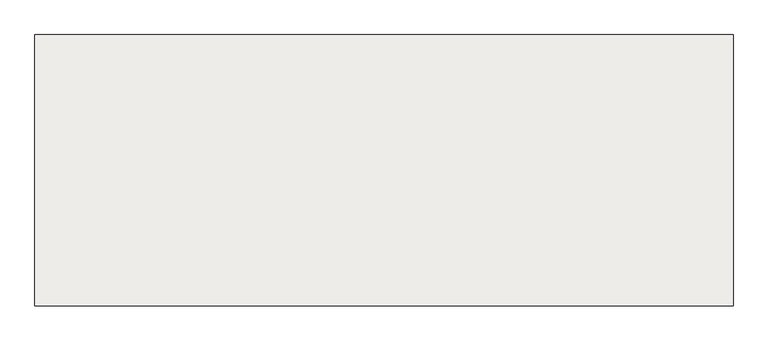
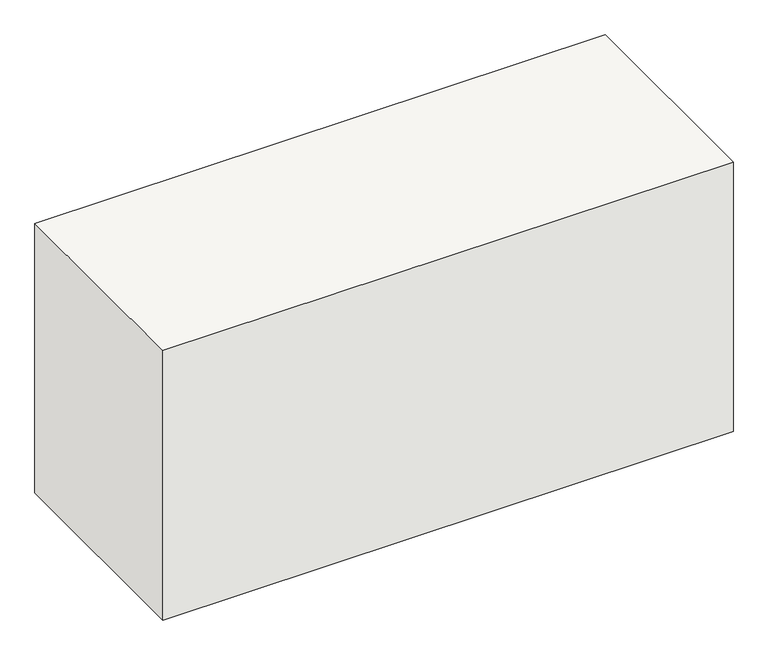
"""IFC4 building model written with IfcOpenShell, lengths in millimetres: footing geometry, NLRS_16_SFO_LB_funderingspoer meerpaals beton ihwg-MMBC-SH_gen_rsf : funderingspoer beton ihwg_gen__2-paals bxlxh 700x1800x1200."""

from ifc_helpers import new_model, si_unit, frame, origin, place, context, project, spatial, polyline, outline, extrude, source, transform, mapped, element, save


def footing_ec8fc613(model_context):
    return source(origin(), model_context, "Body", "SweptSolid", [
        extrude(outline(polyline([(900.0, 350.0), (900.0, -350.0), (-900.0, -350.0), (-900.0, 350.0), (900.0, 350.0)])), frame((0.0, 0.0, -1200.0), z_axis=(0.0, 0.0, 1.0), x_axis=(1.0, 0.0, 0.0)), (0.0, 0.0, 1.0), 900.0),
    ])


if __name__ == "__main__":
    model = new_model("IFC4")
    model_context = context("Model", 3, world=origin())
    ifc_project = project(units=[si_unit("LENGTHUNIT", "METRE", prefix="MILLI")], contexts=[model_context])
    site = spatial("IfcSite", under=ifc_project)
    building = spatial("IfcBuilding", under=site)
    placement = place(None, origin())
    footing_shape = footing_ec8fc613(model_context)
    element("IfcFooting", 1, ObjectType="NLRS_16_SFO_LB_funderingspoer meerpaals beton ihwg-MMBC-SH_gen_rsf : funderingspoer beton ihwg_gen__2-paals bxlxh 700x1800x1200", at=placement, inside=building, context=model_context, shape_type="MappedRepresentation", body=[
        mapped(footing_shape, transform((0.0, 0.0, 0.0), x_axis=(1.0, 0.0, 0.0), y_axis=(0.0, 1.0, 0.0), z_axis=(0.0, 0.0, 1.0))),
    ])
    save(model, "model.ifc")

# Revit data of these elements
# Type "NLRS_16_SFO_LB_funderingspoer meerpaals beton ihwg-MMBC-SH_gen_rsf : funderingspoer beton ihwg_gen__2-paals bxlxh 700x1800x1200"
#   IfcExportAs = "IfcFootingType"
#   Type Comments = "2-paals poer 700x1800x1200"
#   Model = " "
#   Manufacturer = " "
#   Description = "2-paals poer 700x1800x1200"
#   Assembly Code = "16.13"
#   Width = 700 mm
#   Rough Height = 1200 mm
#   NLRS_C_lengte = 1800 mm
#   NLRS_C_hoogte = 1200 mm
#   NLRS_C_breedte = 700 mm
#   Length = 1800 mm
#   Height [instance default] = 1050 mm
#   Foundation Thickness = 1200 mm
#   Depth [instance default] = 150 mm
#   Structural Material = NLRS_f2_beton ihwg_gen_rsf
#   Keynote = ""
# Element 1 (IfcFooting, "NLRS_16_SFO_LB_funderingspoer meerpaals beton ihwg-MMBC-SH_gen_rsf : funderingspoer beton ihwg_gen__2-paals bxlxh 700x1800x1200")
#   Height = 900 mm
#   Depth = 300 mm
#   Materials on its faces: "NLRS_f2_beton ihwg_gen_rsf"
# Materials
#   "NLRS_f2_beton ihwg_gen_rsf": class "F - Niet gebakken kunststeen", colour RGB 129 133 118, transparency 0, Keynote = "f2", Manufacturer = "Revit Standards Foundation", URL = "www.revitstandards.org", Description = "beton ihwg", Cost = 0
